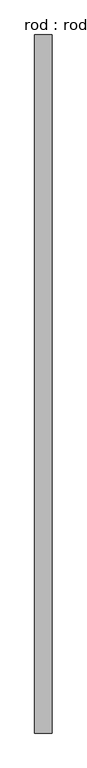
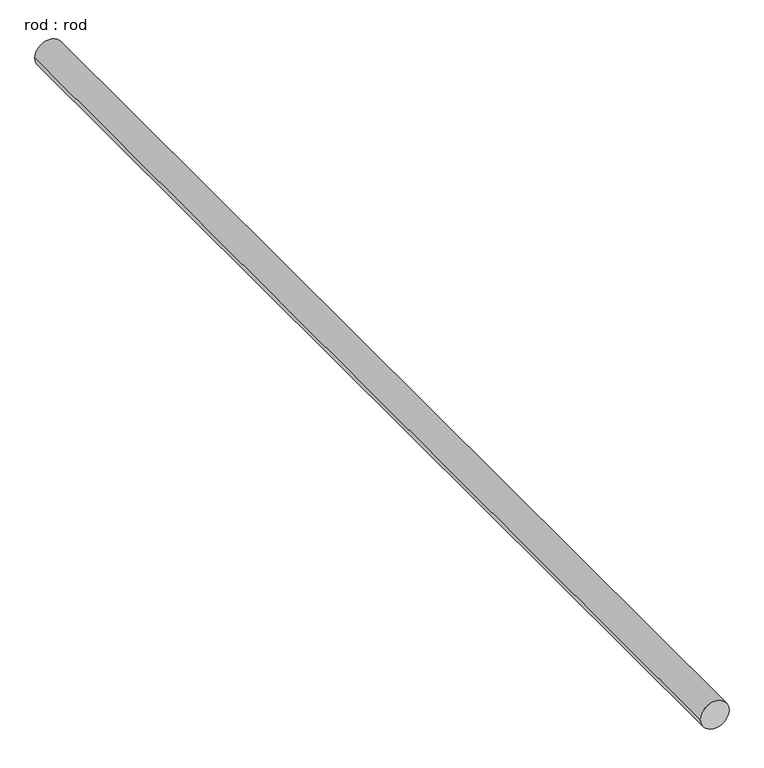
"""IFC4 building model written with IfcOpenShell, lengths in millimetres: proxy geometry, rod : rod."""

from ifc_helpers import new_model, si_unit, point, frame, frame_2d, origin, place, context, project, spatial, circle_curve, trimmed, segment, composite_curve, outline, extrude, source, transform, mapped, element, save


def rod_rod_e209b654(model_context):
    return source(origin(), model_context, "Body", "SweptSolid", [
        extrude(outline(composite_curve([segment(trimmed(circle_curve(frame_2d((0.0108462, 0.0)), 200.0), [point((0.0108462, 200.0))], [point((0.0108462, -200.0))], False, "CARTESIAN"), True, "CONTINUOUS"), segment(trimmed(circle_curve(frame_2d((0.0108462, 0.0)), 200.0), [point((0.0108462, -200.0))], [point((0.0108462, 200.0))], False, "CARTESIAN"), True, "CONTINUOUS")], self_intersect=False)), frame((0.0, -3962.8269402, 0.0), z_axis=(0.0, 1.0, 0.0), x_axis=(0.0, 0.0, 1.0)), (0.0, 0.0, 1.0), 16111.1111111),
    ])


if __name__ == "__main__":
    model = new_model("IFC4")
    model_context = context("Model", 3, world=origin())
    ifc_project = project(units=[si_unit("LENGTHUNIT", "METRE", prefix="MILLI")], contexts=[model_context])
    site = spatial("IfcSite", under=ifc_project)
    building = spatial("IfcBuilding", under=site)
    placement = place(None, origin())
    rod_rod_shape = rod_rod_e209b654(model_context)
    element("IfcBuildingElementProxy", 1, Name="rod : rod", ObjectType="rod : rod", at=placement, inside=building, context=model_context, shape_type="MappedRepresentation", body=[
        mapped(rod_rod_shape, transform((0.0, 0.0, 0.0), x_axis=(1.0, 0.0, 0.0), y_axis=(0.0, 1.0, 0.0), z_axis=(0.0, 0.0, 1.0))),
    ])
    save(model, "model.ifc")

# Revit data of these elements
# Type "rod : rod"
#   Default Elevation = 0
